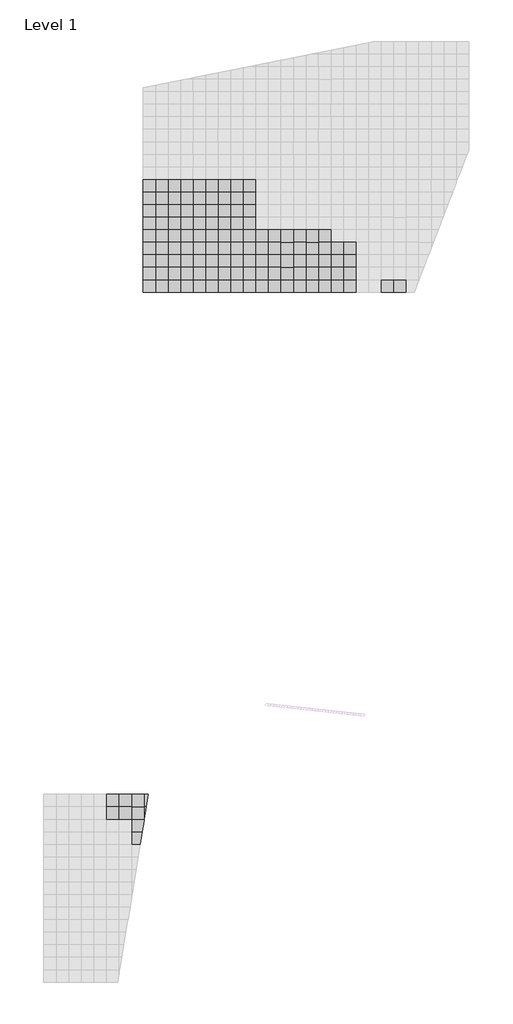
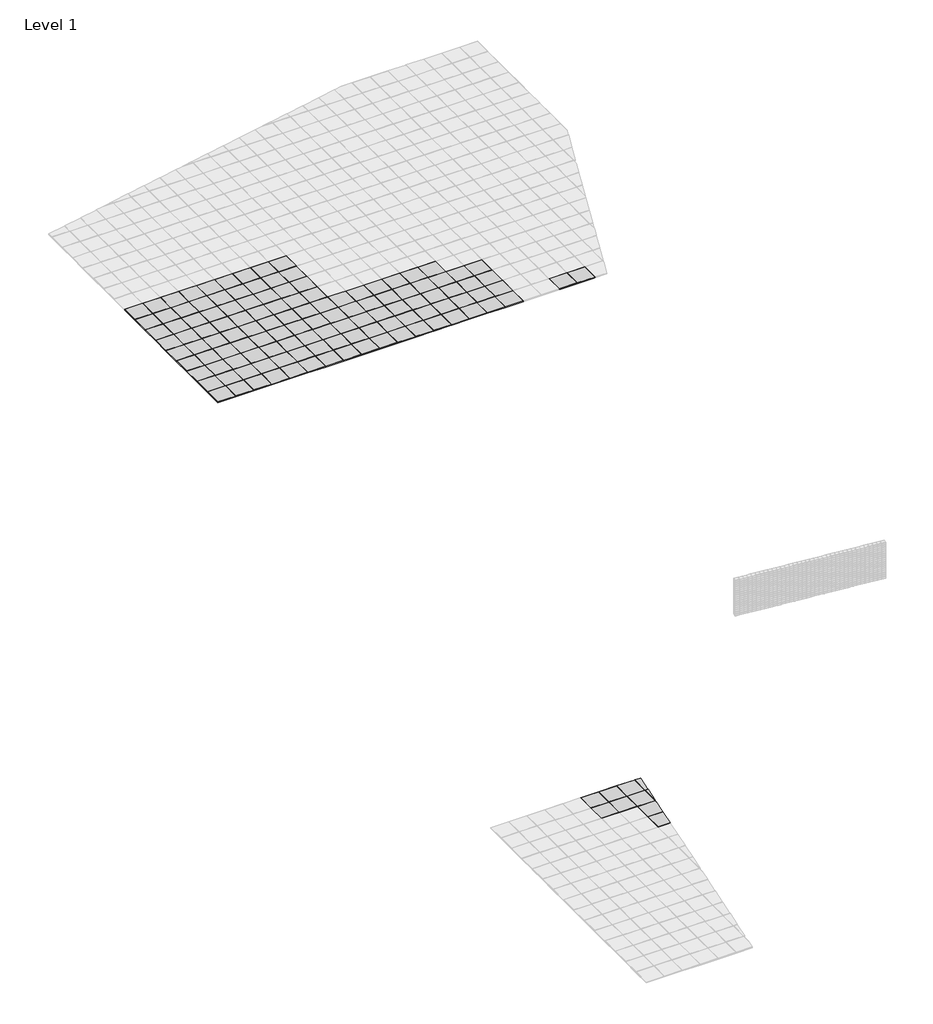
# One storey, part 3 of 18: 131 plates.
# Revit data of these elements (continued)
# Element 5 (IfcPlate, "00_CPA_tegel : Type 1")
#   Area = 0.037868 m²
#   Phase Created = New Construction
#   Materials on its faces: "20_voeg", "300_hardsteen_zwart"
# Elements 6, 7, 8, 9, 10, 11, 12, 13, 14, 15, 16, 17, 18, 19, 20, 21, 22, 23, 24, 25, 26, 27, 28, 29, 30, 31, 32, 33, 34, 35, 36, 37, 38, 39, 40, 41, 42, 43, 44, 45, 46, 47, 48, 49, 50, 51, 52, 53, 54, 55, 56, 57, 58, 59, 60, 61, 62, 63, 64, 65, 66, 67, 68, 69, 70, 71, 72, 73, 74, 75, 76, 77, 78, 79, 80, 81, 82, 83, 84, 85, 86, 87, 88, 89, 90, 91, 92, 93, 94, 95, 96, 97, 98, 99, 100, 101, 102, 103, 104, 105, 106, 107, 108, 109, 110, 111, 112, 113, 114, 115, 116, 117, 118, 119, 120, 121, 122, 123, 124, 125, 126, 127, 128, 129, 130, 131 (IfcPlate, "00_CPA_tegel : Type 1")
#   Area = 0.25 m²
#   Phase Created = New Construction
#   Materials on its faces: "20_voeg", "300_hardsteen_zwart"
# Materials
#   "20_voeg": class "Concrete", colour RGB 86 86 86, transparency 0, Manufacturer = "RevitGG", URL = "www.revitgg.nl", Description = "zandcement, generiek materiaal", Cost = 0
#   "300_hardsteen_zwart": class "Generic", colour RGB 15 15 15, transparency 0, Description = "kalkzandsteen", Cost = 0
